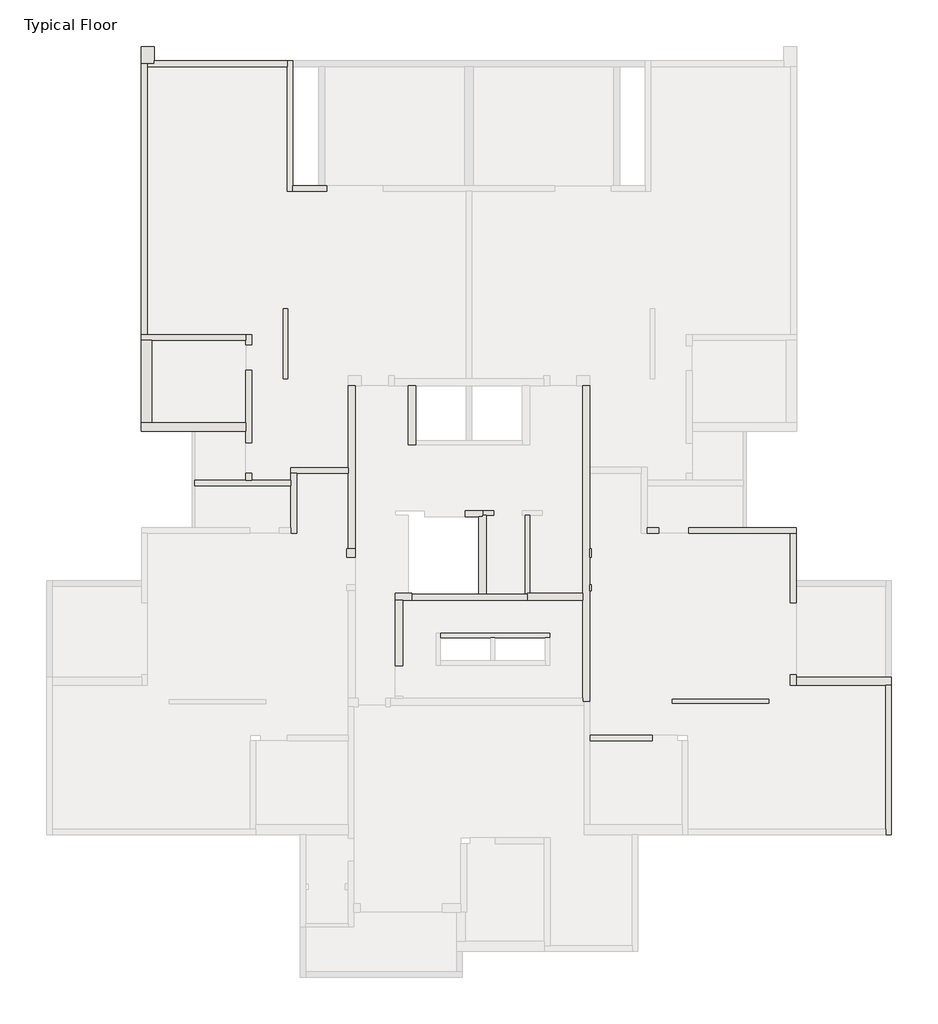
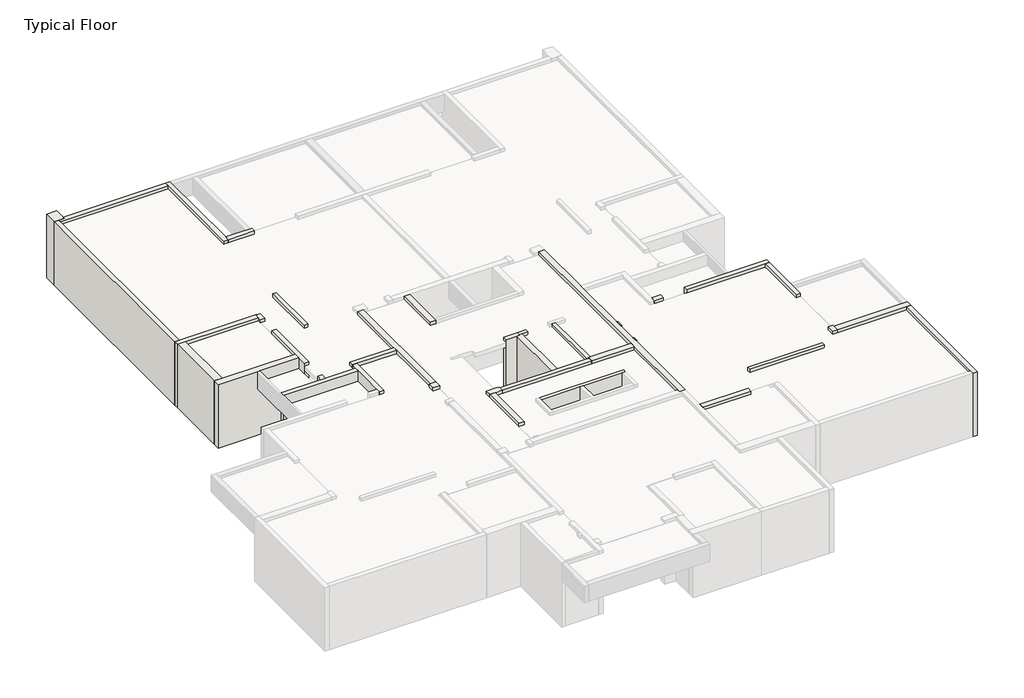
# One storey, part 2 of 4: 38 walls.
"""IFC4 building model written with IfcOpenShell, lengths in millimetres."""

from ifc_helpers import new_model, si_unit, origin, place, context, project, spatial, faceted_brep, element, save

model = new_model("IFC4")

# Units and contexts
model_context = context("Model", 3, world=origin())
ifc_project = project(units=[si_unit("LENGTHUNIT", "METRE", prefix="MILLI")], contexts=[model_context])

# Site, building, storey
site = spatial("IfcSite", under=ifc_project)
building = spatial("IfcBuilding", under=site)
storey = spatial("IfcBuildingStorey", under=building, Name="Typical Floor", Elevation=3160.0)

# Walls
placement = place(None, origin())
element("IfcWall", 1, ObjectType="15", at=placement, inside=storey, context=model_context, shape_type="Brep", body=[
    faceted_brep([(-1883.8880254, 7281.591066, 160.0), (-1883.8880254, 4865.5631538, 160.0), (-1883.8880254, 4865.5631538, 2810.0), (-1883.8880254, 4865.5631538, 3010.0), (-1883.8880254, 4865.5631538, 3160.0), (-1883.8880254, 7281.591066, 3160.0), (-1883.8880254, 7281.591066, 3010.0), (-1883.8880254, 7281.591066, 2810.0), (-1733.8880254, 7281.591066, 160.0), (-1733.8880254, 7281.591066, 2810.0), (-1733.8880254, 7281.591066, 3010.0), (-1733.8880254, 7281.591066, 3160.0), (-1733.8880254, 4865.5631538, 3160.0), (-1733.8880254, 4865.5631538, 3010.0), (-1733.8880254, 4865.5631538, 2810.0), (-1733.8880254, 4865.5631538, 160.0)], [[[0, 1, 2, 3, 4, 5, 6, 7]], [[8, 9, 10, 11, 12, 13, 14, 15]], [[1, 0, 8, 15]], [[4, 3, 2, 1, 15, 14, 13, 12]], [[5, 4, 12, 11]], [[0, 7, 6, 5, 11, 10, 9, 8]]]),
])
element("IfcWall", 2, ObjectType="15", at=placement, inside=storey, context=model_context, shape_type="Brep", body=[
    faceted_brep([(6609.8903055, -2526.1363023, 160.0), (6609.8903055, 156.3601755, 160.0), (6609.8903055, 156.3601755, 2810.0), (6609.8903055, 156.3601755, 3010.0), (6609.8903055, 156.3601755, 3160.0), (6609.8903055, -2526.1363023, 3160.0), (6609.8903055, -2526.1363023, 3010.0), (6609.8903055, -2526.1363023, 2810.0), (6459.8903055, -2576.1363023, 160.0), (6459.8903055, -2576.1363023, 2810.0), (6459.8903055, -2576.1363023, 3010.0), (6459.8903055, -2576.1363023, 3160.0), (6459.8903055, 156.3601755, 3160.0), (6459.8903055, 156.3601755, 3010.0), (6459.8903055, 156.3601755, 2810.0), (6459.8903055, 156.3601755, 160.0), (6534.8903055, -2526.1363023, 160.0), (6534.8903055, -2576.1363023, 160.0), (6534.8903055, -2576.1363023, 3160.0), (6534.8903055, -2526.1363023, 3160.0)], [[[0, 1, 2, 3, 4, 5, 6, 7]], [[8, 9, 10, 11, 12, 13, 14, 15]], [[1, 0, 16, 17, 8, 15]], [[5, 4, 12, 11, 18, 19]], [[0, 7, 6, 5, 19, 16]], [[19, 18, 17, 16]], [[18, 11, 10, 9, 8, 17]], [[4, 3, 2, 1, 15, 14, 13, 12]]]),
])
element("IfcWall", 3, ObjectType="15", at=placement, inside=storey, context=model_context, shape_type="Brep", body=[
    faceted_brep([(11536.8984681, -6331.4817686, 160.0), (14866.281411, -6331.4817686, 160.0), (14866.281411, -6331.4817686, 2810.0), (14866.281411, -6331.4817686, 3010.0), (14866.281411, -6331.4817686, 3160.0), (11536.8984681, -6331.4817686, 3160.0), (11536.8984681, -6331.4817686, 3010.0), (11536.8984681, -6331.4817686, 2810.0), (11536.8984681, -6181.4817686, 160.0), (11536.8984681, -6181.4817686, 2810.0), (11536.8984681, -6181.4817686, 3010.0), (11536.8984681, -6181.4817686, 3160.0), (14866.281411, -6181.4817686, 3160.0), (14866.281411, -6181.4817686, 3010.0), (14866.281411, -6181.4817686, 2810.0), (14866.281411, -6181.4817686, 160.0)], [[[0, 1, 2, 3, 4, 5, 6, 7]], [[8, 9, 10, 11, 12, 13, 14, 15]], [[1, 0, 8, 15]], [[4, 3, 2, 1, 15, 14, 13, 12]], [[5, 4, 12, 11]], [[0, 7, 6, 5, 11, 10, 9, 8]]]),
])
element("IfcWall", 4, ObjectType="15", at=placement, inside=storey, context=model_context, shape_type="Brep", body=[
    faceted_brep([(3535.5549057, -4065.4538564, 160.0), (5268.6420666, -4065.4538564, 160.0), (5418.6420666, -4065.4538564, 160.0), (7154.2538596, -4065.4538564, 160.0), (7304.2538596, -4065.4538564, 160.0), (7304.2538596, -4065.4538564, 3160.0), (7154.2538596, -4065.4538564, 3160.0), (5418.6420666, -4065.4538564, 3160.0), (5268.6420666, -4065.4538564, 3160.0), (3535.5549057, -4065.4538564, 3160.0), (3535.5549057, -3915.4538564, 160.0), (3535.5549057, -3915.4538564, 3160.0), (7304.2538596, -3915.4538564, 3160.0), (7304.2538596, -3915.4538564, 3010.0), (7304.2538596, -3915.4538564, 2810.0), (7304.2538596, -3915.4538564, 160.0)], [[[0, 1, 2, 3, 4, 5, 6, 7, 8, 9]], [[10, 11, 12, 13, 14, 15]], [[4, 3, 2, 1, 0, 10, 15]], [[9, 8, 7, 6, 5, 12, 11]], [[0, 9, 11, 10]], [[5, 4, 15, 14, 13, 12]]]),
])
element("IfcWall", 5, ObjectType="15", at=placement, inside=storey, context=model_context, shape_type="Brep", body=[
    faceted_brep([(4991.7132216, 156.3601755, 160.0), (5116.7132216, 156.3601755, 160.0), (5376.7132216, 156.3601755, 160.0), (5376.7132216, 156.3601755, 2810.0), (5376.7132216, 156.3601755, 3010.0), (5376.7132216, 156.3601755, 3160.0), (5116.7132216, 156.3601755, 3160.0), (4991.7132216, 156.3601755, 3160.0), (4991.7132216, 306.3601755, 160.0), (4991.7132216, 306.3601755, 3160.0), (5376.7132216, 306.3601755, 3160.0), (5376.7132216, 306.3601755, 3010.0), (5376.7132216, 306.3601755, 2810.0), (5376.7132216, 306.3601755, 160.0)], [[[0, 1, 2, 3, 4, 5, 6, 7]], [[8, 9, 10, 11, 12, 13]], [[2, 1, 0, 8, 13]], [[5, 4, 3, 2, 13, 12, 11, 10]], [[7, 6, 5, 10, 9]], [[0, 7, 9, 8]]]),
])
element("IfcWall", 6, ObjectType="20", at=placement, inside=storey, context=model_context, shape_type="Brep", body=[
    faceted_brep([(-6774.1013669, 15724.626844, 160.0), (-6774.1013669, 6387.8215778, 160.0), (-6774.1013669, 6387.8215778, 3160.0), (-6774.1013669, 15724.626844, 3160.0), (-6574.1013669, 15724.626844, 160.0), (-6574.1013669, 15724.626844, 3160.0), (-6574.1013669, 15624.626844, 3160.0), (-6574.1013669, 6387.8215778, 3160.0), (-6574.1013669, 6387.8215778, 3010.0), (-6574.1013669, 6387.8215778, 2810.0), (-6574.1013669, 6387.8215778, 160.0), (-6574.1013669, 15624.626844, 160.0)], [[[0, 1, 2, 3]], [[4, 5, 6, 7, 8, 9, 10, 11]], [[1, 0, 4, 11, 10]], [[3, 2, 7, 6, 5]], [[0, 3, 5, 4]], [[2, 1, 10, 9, 8, 7]]]),
])
element("IfcWall", 7, ObjectType="20", at=placement, inside=storey, context=model_context, shape_type="Brep", body=[
    faceted_brep([(-6774.1013669, 6187.8215778, 160.0), (-6424.1013669, 6187.8215778, 160.0), (-3168.7557226, 6187.8215778, 160.0), (-3168.7557226, 6187.8215778, 2810.0), (-3168.7557226, 6187.8215778, 3010.0), (-3168.7557226, 6187.8215778, 3160.0), (-6424.1013669, 6187.8215778, 3160.0), (-6774.1013669, 6187.8215778, 3160.0), (-6774.1013669, 6387.8215778, 160.0), (-6774.1013669, 6387.8215778, 3160.0), (-6574.1013669, 6387.8215778, 3160.0), (-3168.7557226, 6387.8215778, 3160.0), (-3168.7557226, 6387.8215778, 160.0), (-6574.1013669, 6387.8215778, 160.0)], [[[0, 1, 2, 3, 4, 5, 6, 7]], [[8, 9, 10, 11, 12, 13]], [[2, 1, 0, 8, 13, 12]], [[7, 6, 5, 11, 10, 9]], [[0, 7, 9, 8]], [[5, 4, 3, 2, 12, 11]]]),
])
element("IfcWall", 8, ObjectType="20", at=placement, inside=storey, context=model_context, shape_type="Brep", body=[
    faceted_brep([(-3168.7557226, 1604.6693841, 160.0), (-3168.7557226, 1364.6693841, 160.0), (-3168.7557226, 1364.6693841, 2510.0), (-3168.7557226, 1364.6693841, 2660.0), (-3168.7557226, 1364.6693841, 3160.0), (-3168.7557226, 1604.6693841, 3160.0), (-3168.7557226, 1604.6693841, 3010.0), (-3168.7557226, 1604.6693841, 2810.0), (-2968.7557226, 1604.6693841, 160.0), (-2968.7557226, 1604.6693841, 2810.0), (-2968.7557226, 1604.6693841, 3010.0), (-2968.7557226, 1604.6693841, 3160.0), (-2968.7557226, 1364.6693841, 3160.0), (-2968.7557226, 1364.6693841, 3010.0), (-2968.7557226, 1364.6693841, 2810.0), (-2968.7557226, 1364.6693841, 160.0)], [[[0, 1, 2, 3, 4, 5, 6, 7]], [[8, 9, 10, 11, 12, 13, 14, 15]], [[1, 0, 8, 15]], [[5, 4, 12, 11]], [[0, 7, 6, 5, 11, 10, 9, 8]], [[4, 3, 2, 1, 15, 14, 13, 12]]]),
])
element("IfcWall", 9, ObjectType="20", at=placement, inside=storey, context=model_context, shape_type="Brep", body=[
    faceted_brep([(-1618.0126357, 1364.6693841, 160.0), (-2968.7557226, 1364.6693841, 160.0), (-3168.7557226, 1364.6693841, 160.0), (-4927.8090865, 1364.6693841, 160.0), (-4927.8090865, 1364.6693841, 2510.0), (-4927.8090865, 1364.6693841, 2660.0), (-4927.8090865, 1364.6693841, 3160.0), (-3168.7557226, 1364.6693841, 3160.0), (-2968.7557226, 1364.6693841, 3160.0), (-1618.0126357, 1364.6693841, 3160.0), (-1618.0126357, 1364.6693841, 3010.0), (-1618.0126357, 1364.6693841, 2810.0), (-1618.0126357, 1164.6693841, 160.0), (-1618.0126357, 1164.6693841, 2510.0), (-1618.0126357, 1164.6693841, 2660.0), (-1618.0126357, 1164.6693841, 3160.0), (-4927.8090865, 1164.6693841, 3160.0), (-4927.8090865, 1164.6693841, 2660.0), (-4927.8090865, 1164.6693841, 2510.0), (-4927.8090865, 1164.6693841, 160.0)], [[[0, 1, 2, 3, 4, 5, 6, 7, 8, 9, 10, 11]], [[12, 13, 14, 15, 16, 17, 18, 19]], [[3, 2, 1, 0, 12, 19]], [[6, 5, 4, 3, 19, 18, 17, 16]], [[9, 8, 7, 6, 16, 15]], [[0, 11, 10, 9, 15, 14, 13, 12]]]),
])
element("IfcWall", 10, ObjectType="20", at=placement, inside=storey, context=model_context, shape_type="Brep", body=[
    faceted_brep([(-1750.9499448, 15824.626844, 160.0), (-1750.9499448, 15624.626844, 160.0), (-1750.9499448, 11324.9195447, 160.0), (-1750.9499448, 11324.9195447, 2810.0), (-1750.9499448, 11324.9195447, 3010.0), (-1750.9499448, 11324.9195447, 3160.0), (-1750.9499448, 15624.626844, 3160.0), (-1750.9499448, 15824.626844, 3160.0), (-1550.9499448, 15824.626844, 160.0), (-1550.9499448, 15824.626844, 3160.0), (-1550.9499448, 11524.9195447, 3160.0), (-1550.9499448, 11324.9195447, 3160.0), (-1550.9499448, 11324.9195447, 160.0), (-1550.9499448, 11524.9195447, 160.0)], [[[0, 1, 2, 3, 4, 5, 6, 7]], [[8, 9, 10, 11, 12, 13]], [[2, 1, 0, 8, 13, 12]], [[7, 6, 5, 11, 10, 9]], [[0, 7, 9, 8]], [[5, 4, 3, 2, 12, 11]]]),
])
element("IfcWall", 11, ObjectType="20", at=placement, inside=storey, context=model_context, shape_type="Brep", body=[
    faceted_brep([(-1750.9499448, 15824.626844, 160.0), (-6324.1013669, 15824.626844, 160.0), (-6324.1013669, 15824.626844, 3160.0), (-1750.9499448, 15824.626844, 3160.0), (-1750.9499448, 15624.626844, 160.0), (-1750.9499448, 15624.626844, 2810.0), (-1750.9499448, 15624.626844, 3010.0), (-1750.9499448, 15624.626844, 3160.0), (-6574.1013669, 15624.626844, 3160.0), (-6574.1013669, 15624.626844, 3010.0), (-6574.1013669, 15624.626844, 2810.0), (-6574.1013669, 15624.626844, 160.0), (-6574.1013669, 15724.626844, 160.0), (-6324.1013669, 15724.626844, 160.0), (-6324.1013669, 15724.626844, 3160.0), (-6574.1013669, 15724.626844, 3160.0)], [[[0, 1, 2, 3]], [[4, 5, 6, 7, 8, 9, 10, 11]], [[1, 0, 4, 11, 12, 13]], [[3, 2, 14, 15, 8, 7]], [[0, 3, 7, 6, 5, 4]], [[2, 1, 13, 14]], [[13, 12, 15, 14]], [[12, 11, 10, 9, 8, 15]]]),
])
element("IfcWall", 12, ObjectType="20", at=placement, inside=storey, context=model_context, shape_type="Brep", body=[
    faceted_brep([(15808.1220541, -271.5348131, 160.0), (12108.1220541, -271.5348131, 160.0), (12108.1220541, -271.5348131, 2510.0), (12108.1220541, -271.5348131, 2660.0), (12108.1220541, -271.5348131, 3160.0), (15808.1220541, -271.5348131, 3160.0), (15808.1220541, -471.5348131, 160.0), (15808.1220541, -471.5348131, 3160.0), (15608.1220541, -471.5348131, 3160.0), (12108.1220541, -471.5348131, 3160.0), (12108.1220541, -471.5348131, 2660.0), (12108.1220541, -471.5348131, 2510.0), (12108.1220541, -471.5348131, 160.0), (15608.1220541, -471.5348131, 160.0)], [[[0, 1, 2, 3, 4, 5]], [[6, 7, 8, 9, 10, 11, 12, 13]], [[1, 0, 6, 13, 12]], [[4, 3, 2, 1, 12, 11, 10, 9]], [[5, 4, 9, 8, 7]], [[0, 5, 7, 6]]]),
])
element("IfcWall", 13, ObjectType="20", at=placement, inside=storey, context=model_context, shape_type="Brep", body=[
    faceted_brep([(15608.1220541, -5351.6580536, 160.0), (15608.1220541, -5711.5348131, 160.0), (15608.1220541, -5711.5348131, 2810.0), (15608.1220541, -5711.5348131, 3010.0), (15608.1220541, -5711.5348131, 3160.0), (15608.1220541, -5351.6580536, 3160.0), (15608.1220541, -5351.6580536, 3010.0), (15608.1220541, -5351.6580536, 2810.0), (15808.1220541, -5351.6580536, 160.0), (15808.1220541, -5351.6580536, 2810.0), (15808.1220541, -5351.6580536, 3010.0), (15808.1220541, -5351.6580536, 3160.0), (15808.1220541, -5431.5348131, 3160.0), (15808.1220541, -5711.5348131, 3160.0), (15808.1220541, -5711.5348131, 160.0), (15808.1220541, -5431.5348131, 160.0)], [[[0, 1, 2, 3, 4, 5, 6, 7]], [[8, 9, 10, 11, 12, 13, 14, 15]], [[1, 0, 8, 15, 14]], [[5, 4, 13, 12, 11]], [[0, 7, 6, 5, 11, 10, 9, 8]], [[4, 3, 2, 1, 14, 13]]]),
])
element("IfcWall", 14, ObjectType="20", at=placement, inside=storey, context=model_context, shape_type="Brep", body=[
    faceted_brep([(18889.4302812, -5711.5348131, 160.0), (18889.4302812, -10669.1739201, 160.0), (18889.4302812, -10869.1739201, 160.0), (18889.4302812, -10869.1739201, 3160.0), (18889.4302812, -10669.1739201, 3160.0), (18889.4302812, -5711.5348131, 3160.0), (18889.4302812, -5711.5348131, 3010.0), (18889.4302812, -5711.5348131, 2810.0), (19089.4302812, -5711.5348131, 160.0), (19089.4302812, -5711.5348131, 3160.0), (19089.4302812, -10869.1739201, 3160.0), (19089.4302812, -10869.1739201, 160.0)], [[[0, 1, 2, 3, 4, 5, 6, 7]], [[8, 9, 10, 11]], [[2, 1, 0, 8, 11]], [[5, 4, 3, 10, 9]], [[0, 7, 6, 5, 9, 8]], [[3, 2, 11, 10]]]),
])
element("IfcWall", 15, ObjectType="20", at=placement, inside=storey, context=model_context, shape_type="Brep", body=[
    faceted_brep([(10849.2361919, -7425.251138, 160.0), (8689.2361919, -7425.251138, 160.0), (8689.2361919, -7425.251138, 2810.0), (8689.2361919, -7425.251138, 3010.0), (8689.2361919, -7425.251138, 3160.0), (10849.2361919, -7425.251138, 3160.0), (10849.2361919, -7425.251138, 3010.0), (10849.2361919, -7425.251138, 2810.0), (10849.2361919, -7625.251138, 160.0), (10849.2361919, -7625.251138, 2810.0), (10849.2361919, -7625.251138, 3010.0), (10849.2361919, -7625.251138, 3160.0), (8689.2361919, -7625.251138, 3160.0), (8689.2361919, -7625.251138, 3010.0), (8689.2361919, -7625.251138, 2810.0), (8689.2361919, -7625.251138, 160.0)], [[[0, 1, 2, 3, 4, 5, 6, 7]], [[8, 9, 10, 11, 12, 13, 14, 15]], [[1, 0, 8, 15]], [[5, 4, 12, 11]], [[0, 7, 6, 5, 11, 10, 9, 8]], [[4, 3, 2, 1, 15, 14, 13, 12]]]),
])
element("IfcWall", 16, ObjectType="20", at=placement, inside=storey, context=model_context, shape_type="Brep", body=[
    faceted_brep([(8689.2361919, -2440.6761415, 160.0), (8740.4562765, -2440.6761415, 160.0), (8740.4562765, -2440.6761415, 2810.0), (8740.4562765, -2440.6761415, 3010.0), (8740.4562765, -2440.6761415, 3160.0), (8689.2361919, -2440.6761415, 3160.0), (8689.2361919, -2440.6761415, 3010.0), (8689.2361919, -2440.6761415, 2810.0), (8689.2361919, -2240.6761415, 160.0), (8689.2361919, -2240.6761415, 2810.0), (8689.2361919, -2240.6761415, 3010.0), (8689.2361919, -2240.6761415, 3160.0), (8740.4562765, -2240.6761415, 3160.0), (8740.4562765, -2240.6761415, 3010.0), (8740.4562765, -2240.6761415, 2810.0), (8740.4562765, -2240.6761415, 160.0)], [[[0, 1, 2, 3, 4, 5, 6, 7]], [[8, 9, 10, 11, 12, 13, 14, 15]], [[1, 0, 8, 15]], [[4, 3, 2, 1, 15, 14, 13, 12]], [[5, 4, 12, 11]], [[0, 7, 6, 5, 11, 10, 9, 8]]]),
])
element("IfcWall", 17, ObjectType="20", at=placement, inside=storey, context=model_context, shape_type="Brep", body=[
    faceted_brep([(6534.8903055, -2576.1363023, 160.0), (6459.8903055, -2576.1363023, 160.0), (5116.7132216, -2576.1363023, 160.0), (4866.7132216, -2576.1363023, 160.0), (2556.6955539, -2576.1363023, 160.0), (2556.6955539, -2576.1363023, 3160.0), (2681.6955539, -2576.1363023, 3160.0), (4866.7132216, -2576.1363023, 3160.0), (5116.7132216, -2576.1363023, 3160.0), (6459.8903055, -2576.1363023, 3160.0), (6534.8903055, -2576.1363023, 3160.0), (6534.8903055, -2776.1363023, 160.0), (6534.8903055, -2776.1363023, 3160.0), (2556.6955539, -2776.1363023, 3160.0), (2556.6955539, -2776.1363023, 160.0)], [[[0, 1, 2, 3, 4, 5, 6, 7, 8, 9, 10]], [[11, 12, 13, 14]], [[4, 3, 2, 1, 0, 11, 14]], [[5, 4, 14, 13]], [[10, 9, 8, 7, 6, 5, 13, 12]], [[0, 10, 12, 11]]]),
])
element("IfcWall", 18, ObjectType="20", at=placement, inside=storey, context=model_context, shape_type="Brep", body=[
    faceted_brep([(4391.7132216, 106.3601755, 160.0), (4866.7132216, 106.3601755, 160.0), (4991.7132216, 106.3601755, 160.0), (4991.7132216, 106.3601755, 3160.0), (4866.7132216, 106.3601755, 3160.0), (4391.7132216, 106.3601755, 3160.0), (4391.7132216, 106.3601755, 3010.0), (4391.7132216, 106.3601755, 2810.0), (4391.7132216, 306.3601755, 160.0), (4391.7132216, 306.3601755, 2810.0), (4391.7132216, 306.3601755, 3010.0), (4391.7132216, 306.3601755, 3160.0), (4991.7132216, 306.3601755, 3160.0), (4991.7132216, 306.3601755, 160.0), (4991.7132216, 156.3601755, 160.0), (4991.7132216, 156.3601755, 3160.0)], [[[0, 1, 2, 3, 4, 5, 6, 7]], [[8, 9, 10, 11, 12, 13]], [[2, 1, 0, 8, 13, 14]], [[3, 2, 14, 13, 12, 15]], [[5, 4, 3, 15, 12, 11]], [[0, 7, 6, 5, 11, 10, 9, 8]]]),
])
element("IfcWall", 19, ObjectType="20", at=placement, inside=storey, context=model_context, shape_type="Brep", body=[
    faceted_brep([(-1618.0126357, 1602.0583306, 160.0), (-1418.0126357, 1602.0583306, 160.0), (353.0602083, 1602.0583306, 160.0), (353.0602083, 1602.0583306, 2810.0), (353.0602083, 1602.0583306, 3010.0), (353.0602083, 1602.0583306, 3160.0), (-1418.0126357, 1602.0583306, 3160.0), (-1618.0126357, 1602.0583306, 3160.0), (-1618.0126357, 1802.0583306, 160.0), (-1618.0126357, 1802.0583306, 2810.0), (-1618.0126357, 1802.0583306, 3010.0), (-1618.0126357, 1802.0583306, 3160.0), (353.0602083, 1802.0583306, 3160.0), (353.0602083, 1802.0583306, 3010.0), (353.0602083, 1802.0583306, 2810.0), (353.0602083, 1802.0583306, 160.0)], [[[0, 1, 2, 3, 4, 5, 6, 7]], [[8, 9, 10, 11, 12, 13, 14, 15]], [[2, 1, 0, 8, 15]], [[7, 6, 5, 12, 11]], [[5, 4, 3, 2, 15, 14, 13, 12]], [[0, 7, 11, 10, 9, 8]]]),
])
element("IfcWall", 20, ObjectType="20", at=placement, inside=storey, context=model_context, shape_type="Brep", body=[
    faceted_brep([(-1618.0126357, 1602.0583306, 160.0), (-1618.0126357, 1364.6693841, 160.0), (-1618.0126357, 1164.6693841, 160.0), (-1618.0126357, -271.5347538, 160.0), (-1618.0126357, -471.5347538, 160.0), (-1618.0126357, -471.5347538, 3160.0), (-1618.0126357, -271.5347538, 3160.0), (-1618.0126357, 1164.6693841, 3160.0), (-1618.0126357, 1364.6693841, 3160.0), (-1618.0126357, 1602.0583306, 3160.0), (-1418.0126357, 1602.0583306, 160.0), (-1418.0126357, 1602.0583306, 2810.0), (-1418.0126357, 1602.0583306, 3010.0), (-1418.0126357, 1602.0583306, 3160.0), (-1418.0126357, -471.5347538, 3160.0), (-1418.0126357, -471.5347538, 3010.0), (-1418.0126357, -471.5347538, 2810.0), (-1418.0126357, -471.5347538, 160.0)], [[[0, 1, 2, 3, 4, 5, 6, 7, 8, 9]], [[10, 11, 12, 13, 14, 15, 16, 17]], [[4, 3, 2, 1, 0, 10, 17]], [[9, 8, 7, 6, 5, 14, 13]], [[5, 4, 17, 16, 15, 14]], [[0, 9, 13, 12, 11, 10]]]),
])
element("IfcWall", 21, ObjectType="20", at=placement, inside=storey, context=model_context, shape_type="Brep", body=[
    faceted_brep([(15808.1220541, -2868.5711301, 160.0), (15808.1220541, -471.5348131, 160.0), (15808.1220541, -471.5348131, 3160.0), (15808.1220541, -2868.5711301, 3160.0), (15808.1220541, -2868.5711301, 3010.0), (15808.1220541, -2868.5711301, 2810.0), (15608.1220541, -2868.5711301, 160.0), (15608.1220541, -2868.5711301, 2810.0), (15608.1220541, -2868.5711301, 3010.0), (15608.1220541, -2868.5711301, 3160.0), (15608.1220541, -471.5348131, 3160.0), (15608.1220541, -471.5348131, 3010.0), (15608.1220541, -471.5348131, 2810.0), (15608.1220541, -471.5348131, 160.0)], [[[0, 1, 2, 3, 4, 5]], [[6, 7, 8, 9, 10, 11, 12, 13]], [[1, 0, 6, 13]], [[3, 2, 10, 9]], [[0, 5, 4, 3, 9, 8, 7, 6]], [[2, 1, 13, 12, 11, 10]]]),
])
element("IfcWall", 22, ObjectType="20", at=placement, inside=storey, context=model_context, shape_type="Brep", body=[
    faceted_brep([(-390.7110009, 11524.9195447, 160.0), (-1550.9499448, 11524.9195447, 160.0), (-1550.9499448, 11524.9195447, 3160.0), (-390.7110009, 11524.9195447, 3160.0), (-390.7110009, 11524.9195447, 3010.0), (-390.7110009, 11524.9195447, 2810.0), (-390.7110009, 11324.9195447, 160.0), (-390.7110009, 11324.9195447, 2810.0), (-390.7110009, 11324.9195447, 3010.0), (-390.7110009, 11324.9195447, 3160.0), (-1550.9499448, 11324.9195447, 3160.0), (-1550.9499448, 11324.9195447, 160.0)], [[[0, 1, 2, 3, 4, 5]], [[6, 7, 8, 9, 10, 11]], [[1, 0, 6, 11]], [[3, 2, 10, 9]], [[0, 5, 4, 3, 9, 8, 7, 6]], [[2, 1, 11, 10]]]),
])
element("IfcWall", 23, ObjectType="20", at=placement, inside=storey, context=model_context, shape_type="Brep", body=[
    faceted_brep([(-2968.7557226, 2648.3506111, 160.0), (-2968.7557226, 5158.3506111, 160.0), (-2968.7557226, 5158.3506111, 2810.0), (-2968.7557226, 5158.3506111, 3010.0), (-2968.7557226, 5158.3506111, 3160.0), (-2968.7557226, 2648.3506111, 3160.0), (-2968.7557226, 2648.3506111, 3010.0), (-2968.7557226, 2648.3506111, 2810.0), (-3168.7557226, 2648.3506111, 160.0), (-3168.7557226, 2648.3506111, 2810.0), (-3168.7557226, 2648.3506111, 3010.0), (-3168.7557226, 2648.3506111, 3160.0), (-3168.7557226, 3048.3506111, 3160.0), (-3168.7557226, 3348.3506111, 3160.0), (-3168.7557226, 5158.3506111, 3160.0), (-3168.7557226, 5158.3506111, 3010.0), (-3168.7557226, 5158.3506111, 2810.0), (-3168.7557226, 5158.3506111, 160.0), (-3168.7557226, 3348.3506111, 160.0), (-3168.7557226, 3048.3506111, 160.0)], [[[0, 1, 2, 3, 4, 5, 6, 7]], [[8, 9, 10, 11, 12, 13, 14, 15, 16, 17, 18, 19]], [[1, 0, 8, 19, 18, 17]], [[4, 3, 2, 1, 17, 16, 15, 14]], [[5, 4, 14, 13, 12, 11]], [[0, 7, 6, 5, 11, 10, 9, 8]]]),
])
element("IfcWall", 24, ObjectType="20", at=placement, inside=storey, context=model_context, shape_type="Brep", body=[
    faceted_brep([(-3168.7557226, 6387.8215778, 160.0), (-3168.7557226, 6187.8215778, 160.0), (-3168.7557226, 6027.8215778, 160.0), (-3168.7557226, 6027.8215778, 2810.0), (-3168.7557226, 6027.8215778, 3010.0), (-3168.7557226, 6027.8215778, 3160.0), (-3168.7557226, 6187.8215778, 3160.0), (-3168.7557226, 6387.8215778, 3160.0), (-2968.7557226, 6387.8215778, 160.0), (-2968.7557226, 6387.8215778, 2810.0), (-2968.7557226, 6387.8215778, 3010.0), (-2968.7557226, 6387.8215778, 3160.0), (-2968.7557226, 6027.8215778, 3160.0), (-2968.7557226, 6027.8215778, 3010.0), (-2968.7557226, 6027.8215778, 2810.0), (-2968.7557226, 6027.8215778, 160.0)], [[[0, 1, 2, 3, 4, 5, 6, 7]], [[8, 9, 10, 11, 12, 13, 14, 15]], [[2, 1, 0, 8, 15]], [[5, 4, 3, 2, 15, 14, 13, 12]], [[7, 6, 5, 12, 11]], [[0, 7, 11, 10, 9, 8]]]),
])
element("IfcWall", 25, ObjectType="20", at=placement, inside=storey, context=model_context, shape_type="Brep", body=[
    faceted_brep([(11062.1205752, -271.5348131, 160.0), (10662.1205752, -271.5348131, 160.0), (10662.1205752, -271.5348131, 2510.0), (10662.1205752, -271.5348131, 2660.0), (10662.1205752, -271.5348131, 3160.0), (11062.1205752, -271.5348131, 3160.0), (11062.1205752, -271.5348131, 2660.0), (11062.1205752, -271.5348131, 2510.0), (11062.1205752, -471.5348131, 160.0), (11062.1205752, -471.5348131, 2510.0), (11062.1205752, -471.5348131, 2660.0), (11062.1205752, -471.5348131, 3160.0), (10662.1205752, -471.5348131, 3160.0), (10662.1205752, -471.5348131, 160.0)], [[[0, 1, 2, 3, 4, 5, 6, 7]], [[8, 9, 10, 11, 12, 13]], [[1, 0, 8, 13]], [[5, 4, 12, 11]], [[0, 7, 6, 5, 11, 10, 9, 8]], [[4, 3, 2, 1, 13, 12]]]),
])
element("IfcWall", 26, ObjectType="25", at=placement, inside=storey, context=model_context, shape_type="Brep", body=[
    faceted_brep([(2434.2185243, 4615.5631538, 160.0), (2434.2185243, 2582.4743311, 160.0), (2434.2185243, 2582.4743311, 2810.0), (2434.2185243, 2582.4743311, 3010.0), (2434.2185243, 2582.4743311, 3160.0), (2434.2185243, 4615.5631538, 3160.0), (2434.2185243, 4615.5631538, 3010.0), (2434.2185243, 4615.5631538, 2810.0), (2684.2185243, 4615.5631538, 160.0), (2684.2185243, 4615.5631538, 3160.0), (2684.2185243, 2732.4743311, 3160.0), (2684.2185243, 2582.4743311, 3160.0), (2684.2185243, 2582.4743311, 160.0), (2684.2185243, 2732.4743311, 160.0)], [[[0, 1, 2, 3, 4, 5, 6, 7]], [[8, 9, 10, 11, 12, 13]], [[1, 0, 8, 13, 12]], [[5, 4, 11, 10, 9]], [[0, 7, 6, 5, 9, 8]], [[4, 3, 2, 1, 12, 11]]]),
])
element("IfcWall", 27, ObjectType="25", at=placement, inside=storey, context=model_context, shape_type="Brep", body=[
    faceted_brep([(8689.2361919, -6275.4733638, 160.0), (8689.2361919, -2440.6761415, 160.0), (8689.2361919, -2240.6761415, 160.0), (8689.2361919, -1298.8355577, 160.0), (8689.2361919, -998.8355577, 160.0), (8689.2361919, 1602.6523966, 160.0), (8689.2361919, 1802.6523966, 160.0), (8689.2361919, 4613.0861241, 160.0), (8689.2361919, 4613.0861241, 3160.0), (8689.2361919, 1802.6523966, 3160.0), (8689.2361919, 1602.6523966, 3160.0), (8689.2361919, -998.8355577, 3160.0), (8689.2361919, -1298.8355577, 3160.0), (8689.2361919, -2240.6761415, 3160.0), (8689.2361919, -2440.6761415, 3160.0), (8689.2361919, -6275.4733638, 3160.0), (8439.2361919, -6275.4733638, 160.0), (8439.2361919, -6275.4733638, 3160.0), (8439.2361919, -6150.4733638, 3160.0), (8439.2361919, -2776.1363023, 3160.0), (8439.2361919, -2526.1363023, 3160.0), (8439.2361919, 4613.0861241, 3160.0), (8439.2361919, 4613.0861241, 3010.0), (8439.2361919, 4613.0861241, 2810.0), (8439.2361919, 4613.0861241, 160.0), (8439.2361919, -2526.1363023, 160.0), (8439.2361919, -2776.1363023, 160.0), (8439.2361919, -6150.4733638, 160.0), (8489.2361919, -6275.4733638, 160.0), (8489.2361919, -6275.4733638, 3160.0)], [[[0, 1, 2, 3, 4, 5, 6, 7, 8, 9, 10, 11, 12, 13, 14, 15]], [[16, 17, 18, 19, 20, 21, 22, 23, 24, 25, 26, 27]], [[7, 6, 5, 4, 3, 2, 1, 0, 28, 16, 27, 26, 25, 24]], [[8, 7, 24, 23, 22, 21]], [[15, 14, 13, 12, 11, 10, 9, 8, 21, 20, 19, 18, 17, 29]], [[0, 15, 29, 17, 16, 28]]]),
])
element("IfcWall", 28, ObjectType="25", at=placement, inside=storey, context=model_context, shape_type="Brep", body=[
    faceted_brep([(8439.2361919, -2526.1363023, 160.0), (6609.8903055, -2526.1363023, 160.0), (6534.8903055, -2526.1363023, 160.0), (6534.8903055, -2526.1363023, 3160.0), (6609.8903055, -2526.1363023, 3160.0), (8439.2361919, -2526.1363023, 3160.0), (8439.2361919, -2526.1363023, 3010.0), (8439.2361919, -2526.1363023, 2810.0), (8439.2361919, -2776.1363023, 160.0), (8439.2361919, -2776.1363023, 3160.0), (6534.8903055, -2776.1363023, 3160.0), (6534.8903055, -2776.1363023, 160.0), (6534.8903055, -2576.1363023, 160.0), (6534.8903055, -2576.1363023, 3160.0)], [[[0, 1, 2, 3, 4, 5, 6, 7]], [[8, 9, 10, 11]], [[2, 1, 0, 8, 11, 12]], [[3, 2, 12, 11, 10, 13]], [[5, 4, 3, 13, 10, 9]], [[0, 7, 6, 5, 9, 8]]]),
])
element("IfcWall", 29, ObjectType="25", at=placement, inside=storey, context=model_context, shape_type="Brep", body=[
    faceted_brep([(4866.7132216, 106.3601755, 160.0), (4866.7132216, -2576.1363023, 160.0), (4866.7132216, -2576.1363023, 3160.0), (4866.7132216, 106.3601755, 3160.0), (5116.7132216, 156.3601755, 160.0), (5116.7132216, 156.3601755, 2810.0), (5116.7132216, 156.3601755, 3010.0), (5116.7132216, 156.3601755, 3160.0), (5116.7132216, -2576.1363023, 3160.0), (5116.7132216, -2576.1363023, 3010.0), (5116.7132216, -2576.1363023, 2810.0), (5116.7132216, -2576.1363023, 160.0), (4991.7132216, 106.3601755, 160.0), (4991.7132216, 156.3601755, 160.0), (4991.7132216, 156.3601755, 3160.0), (4991.7132216, 106.3601755, 3160.0)], [[[0, 1, 2, 3]], [[4, 5, 6, 7, 8, 9, 10, 11]], [[1, 0, 12, 13, 4, 11]], [[3, 2, 8, 7, 14, 15]], [[2, 1, 11, 10, 9, 8]], [[0, 3, 15, 12]], [[15, 14, 13, 12]], [[14, 7, 6, 5, 4, 13]]]),
])
element("IfcWall", 30, ObjectType="25", at=placement, inside=storey, context=model_context, shape_type="Brep", body=[
    faceted_brep([(353.0602083, 4618.0861241, 160.0), (353.0602083, 1802.0583306, 160.0), (353.0602083, 1602.0583306, 160.0), (353.0602083, -998.8355577, 160.0), (353.0602083, -998.8355577, 2810.0), (353.0602083, -998.8355577, 3010.0), (353.0602083, -998.8355577, 3160.0), (353.0602083, 1602.0583306, 3160.0), (353.0602083, 1802.0583306, 3160.0), (353.0602083, 4618.0861241, 3160.0), (603.0602083, 4618.0861241, 160.0), (603.0602083, 4618.0861241, 2810.0), (603.0602083, 4618.0861241, 3010.0), (603.0602083, 4618.0861241, 3160.0), (603.0602083, -998.8355577, 3160.0), (603.0602083, -998.8355577, 160.0)], [[[0, 1, 2, 3, 4, 5, 6, 7, 8, 9]], [[10, 11, 12, 13, 14, 15]], [[3, 2, 1, 0, 10, 15]], [[9, 8, 7, 6, 14, 13]], [[0, 9, 13, 12, 11, 10]], [[6, 5, 4, 3, 15, 14]]]),
])
element("IfcWall", 31, ObjectType="25", at=placement, inside=storey, context=model_context, shape_type="Brep", body=[
    faceted_brep([(2237.3338395, -5031.1363023, 160.0), (2237.3338395, -2776.1363023, 160.0), (2237.3338395, -2776.1363023, 2810.0), (2237.3338395, -2776.1363023, 3010.0), (2237.3338395, -2776.1363023, 3160.0), (2237.3338395, -5031.1363023, 3160.0), (2237.3338395, -5031.1363023, 3010.0), (2237.3338395, -5031.1363023, 2810.0), (1987.3338395, -5031.1363023, 160.0), (1987.3338395, -5031.1363023, 2810.0), (1987.3338395, -5031.1363023, 3010.0), (1987.3338395, -5031.1363023, 3160.0), (1987.3338395, -2776.1363023, 3160.0), (1987.3338395, -2776.1363023, 160.0)], [[[0, 1, 2, 3, 4, 5, 6, 7]], [[8, 9, 10, 11, 12, 13]], [[1, 0, 8, 13]], [[5, 4, 12, 11]], [[0, 7, 6, 5, 11, 10, 9, 8]], [[4, 3, 2, 1, 13, 12]]]),
])
element("IfcWall", 32, ObjectType="25", at=placement, inside=storey, context=model_context, shape_type="Brep", body=[
    faceted_brep([(1987.3338395, -2776.1363023, 160.0), (2237.3338395, -2776.1363023, 160.0), (2556.6955539, -2776.1363023, 160.0), (2556.6955539, -2776.1363023, 3160.0), (2237.3338395, -2776.1363023, 3160.0), (1987.3338395, -2776.1363023, 3160.0), (1987.3338395, -2526.1363023, 160.0), (1987.3338395, -2526.1363023, 2810.0), (1987.3338395, -2526.1363023, 3010.0), (1987.3338395, -2526.1363023, 3160.0), (2431.6955539, -2526.1363023, 3160.0), (2556.6955539, -2526.1363023, 3160.0), (2556.6955539, -2526.1363023, 160.0), (2556.6955539, -2576.1363023, 160.0), (2556.6955539, -2576.1363023, 3160.0)], [[[0, 1, 2, 3, 4, 5]], [[6, 7, 8, 9, 10, 11, 12]], [[2, 1, 0, 6, 12, 13]], [[3, 2, 13, 12, 11, 14]], [[5, 4, 3, 14, 11, 10, 9]], [[0, 5, 9, 8, 7, 6]]]),
])
element("IfcWall", 33, ObjectType="28", at=placement, inside=storey, context=model_context, shape_type="Brep", body=[
    faceted_brep([(15808.1220541, -5711.5348131, 160.0), (18889.4302812, -5711.5348131, 160.0), (19089.4302812, -5711.5348131, 160.0), (19089.4302812, -5711.5348131, 3160.0), (18889.4302812, -5711.5348131, 3160.0), (15808.1220541, -5711.5348131, 3160.0), (15808.1220541, -5431.5348131, 160.0), (15808.1220541, -5431.5348131, 2810.0), (15808.1220541, -5431.5348131, 3010.0), (15808.1220541, -5431.5348131, 3160.0), (19089.4302812, -5431.5348131, 3160.0), (19089.4302812, -5431.5348131, 160.0)], [[[0, 1, 2, 3, 4, 5]], [[6, 7, 8, 9, 10, 11]], [[2, 1, 0, 6, 11]], [[5, 4, 3, 10, 9]], [[0, 5, 9, 8, 7, 6]], [[3, 2, 11, 10]]]),
])
element("IfcWall", 34, ObjectType="30", at=placement, inside=storey, context=model_context, shape_type="Brep", body=[
    faceted_brep([(-3168.7557226, 3348.3506111, 160.0), (-6424.1013669, 3348.3506111, 160.0), (-6774.1013669, 3348.3506111, 160.0), (-6774.1013669, 3348.3506111, 3160.0), (-6424.1013669, 3348.3506111, 3160.0), (-3168.7557226, 3348.3506111, 3160.0), (-3168.7557226, 3348.3506111, 3010.0), (-3168.7557226, 3348.3506111, 2810.0), (-3168.7557226, 3048.3506111, 160.0), (-3168.7557226, 3048.3506111, 2510.0), (-3168.7557226, 3048.3506111, 2660.0), (-3168.7557226, 3048.3506111, 3160.0), (-6774.1013669, 3048.3506111, 3160.0), (-6774.1013669, 3048.3506111, 160.0)], [[[0, 1, 2, 3, 4, 5, 6, 7]], [[8, 9, 10, 11, 12, 13]], [[2, 1, 0, 8, 13]], [[5, 4, 3, 12, 11]], [[3, 2, 13, 12]], [[0, 7, 6, 5, 11, 10, 9, 8]]]),
])
element("IfcWall", 35, ObjectType="30", at=placement, inside=storey, context=model_context, shape_type="Brep", body=[
    faceted_brep([(303.6507728, -1298.8355577, 160.0), (603.0602083, -1298.8355577, 160.0), (603.0602083, -1298.8355577, 2810.0), (603.0602083, -1298.8355577, 3010.0), (603.0602083, -1298.8355577, 3160.0), (303.6507728, -1298.8355577, 3160.0), (303.6507728, -1298.8355577, 3010.0), (303.6507728, -1298.8355577, 2810.0), (303.6507728, -998.8355577, 160.0), (303.6507728, -998.8355577, 2810.0), (303.6507728, -998.8355577, 3010.0), (303.6507728, -998.8355577, 3160.0), (353.0602083, -998.8355577, 3160.0), (603.0602083, -998.8355577, 3160.0), (603.0602083, -998.8355577, 160.0), (353.0602083, -998.8355577, 160.0)], [[[0, 1, 2, 3, 4, 5, 6, 7]], [[8, 9, 10, 11, 12, 13, 14, 15]], [[1, 0, 8, 15, 14]], [[5, 4, 13, 12, 11]], [[0, 7, 6, 5, 11, 10, 9, 8]], [[4, 3, 2, 1, 14, 13]]]),
])
element("IfcWall", 36, ObjectType="30", at=placement, inside=storey, context=model_context, shape_type="Brep", body=[
    faceted_brep([(8689.2361919, -1298.8355577, 160.0), (8740.4562765, -1298.8355577, 160.0), (8740.4562765, -1298.8355577, 2810.0), (8740.4562765, -1298.8355577, 3010.0), (8740.4562765, -1298.8355577, 3160.0), (8689.2361919, -1298.8355577, 3160.0), (8689.2361919, -1298.8355577, 3010.0), (8689.2361919, -1298.8355577, 2810.0), (8689.2361919, -998.8355577, 160.0), (8689.2361919, -998.8355577, 2810.0), (8689.2361919, -998.8355577, 3010.0), (8689.2361919, -998.8355577, 3160.0), (8740.4562765, -998.8355577, 3160.0), (8740.4562765, -998.8355577, 3010.0), (8740.4562765, -998.8355577, 2810.0), (8740.4562765, -998.8355577, 160.0)], [[[0, 1, 2, 3, 4, 5, 6, 7]], [[8, 9, 10, 11, 12, 13, 14, 15]], [[1, 0, 8, 15]], [[4, 3, 2, 1, 15, 14, 13, 12]], [[5, 4, 12, 11]], [[0, 7, 6, 5, 11, 10, 9, 8]]]),
])
element("IfcWall", 37, ObjectType="35", at=placement, inside=storey, context=model_context, shape_type="Brep", body=[
    faceted_brep([(-6424.1013669, 3348.3506111, 160.0), (-6424.1013669, 6187.8215778, 160.0), (-6424.1013669, 6187.8215778, 2810.0), (-6424.1013669, 6187.8215778, 3010.0), (-6424.1013669, 6187.8215778, 3160.0), (-6424.1013669, 3348.3506111, 3160.0), (-6424.1013669, 3348.3506111, 3010.0), (-6424.1013669, 3348.3506111, 2810.0), (-6774.1013669, 3348.3506111, 160.0), (-6774.1013669, 3348.3506111, 3160.0), (-6774.1013669, 6187.8215778, 3160.0), (-6774.1013669, 6187.8215778, 160.0)], [[[0, 1, 2, 3, 4, 5, 6, 7]], [[8, 9, 10, 11]], [[1, 0, 8, 11]], [[5, 4, 10, 9]], [[4, 3, 2, 1, 11, 10]], [[0, 7, 6, 5, 9, 8]]]),
])
element("IfcWall", 38, ObjectType="45", at=placement, inside=storey, context=model_context, shape_type="Brep", body=[
    faceted_brep([(-6774.1013669, 16318.9904575, 160.0), (-6774.1013669, 15724.626844, 160.0), (-6774.1013669, 15724.626844, 3160.0), (-6774.1013669, 16318.9904575, 3160.0), (-6324.1013669, 16318.9904575, 160.0), (-6324.1013669, 16318.9904575, 3160.0), (-6324.1013669, 15824.626844, 3160.0), (-6324.1013669, 15724.626844, 3160.0), (-6324.1013669, 15724.626844, 160.0), (-6324.1013669, 15824.626844, 160.0), (-6574.1013669, 15724.626844, 160.0), (-6574.1013669, 15724.626844, 3160.0)], [[[0, 1, 2, 3]], [[4, 5, 6, 7, 8, 9]], [[1, 0, 4, 9, 8, 10]], [[2, 1, 10, 8, 7, 11]], [[3, 2, 11, 7, 6, 5]], [[0, 3, 5, 4]]]),
])

save(model, "model.ifc")

# Revit data of these elements
# Type "15"
#   Layers, outside or top first: 15 cm "Concrete, Cast-in-Place - B30" (function 1)
# Type "20"
#   Layers, outside or top first: 20 cm "Concrete, Cast-in-Place - B30" (function 1)
# Type "25"
#   Layers, outside or top first: 25 cm "Concrete, Cast-in-Place - B30" (function 1)
# Type "28"
#   Layers, outside or top first: 28 cm "Concrete, Cast-in-Place - B30" (function 1)
# Type "30"
#   Layers, outside or top first: 30 cm "Concrete, Cast-in-Place - B30" (function 1)
# Type "35"
#   Layers, outside or top first: 35 cm "Concrete, Cast-in-Place - B30" (function 1)
# Type "45"
#   Layers, outside or top first: 45 cm "Concrete, Cast-in-Place - B30" (function 1)
# Element 1 (IfcWall, "15")
#   Comments = ""
#   Mark = "W92"
#   SOFiSTiK_AMG_Comments = ""
#   built-in parameter 1001111 = -300 cm
#   Top Offset = 0 cm
#   Base Offset = -300 cm
#   wall height = 300 cm
#   SOFiSTiK_AMG_Scheduled = yes
#   SOFiSTiK_AMG_Adjusted = yes
#   Phase Created = New Construction
#   Base Constraint = Typical Floor
#   Top Constraint = Typical Floor
#   Materials on its faces: "Concrete, Cast-in-Place - B30"
# Element 2 (IfcWall, "15")
#   Comments = ""
#   Mark = "W93"
#   SOFiSTiK_AMG_Comments = ""
#   built-in parameter 1001111 = -300 cm
#   Top Offset = 0 cm
#   Base Offset = -300 cm
#   wall height = 300 cm
#   SOFiSTiK_AMG_Scheduled = yes
#   SOFiSTiK_AMG_Adjusted = yes
#   Phase Created = New Construction
#   Base Constraint = Typical Floor
#   Top Constraint = Typical Floor
#   Materials on its faces: "Concrete, Cast-in-Place - B30"
# Element 3 (IfcWall, "15")
#   Comments = ""
#   Mark = "W97"
#   SOFiSTiK_AMG_Comments = ""
#   built-in parameter 1001111 = -300 cm
#   Top Offset = 0 cm
#   Base Offset = -300 cm
#   wall height = 300 cm
#   SOFiSTiK_AMG_Scheduled = yes
#   SOFiSTiK_AMG_Adjusted = yes
#   Phase Created = New Construction
#   Base Constraint = Typical Floor
#   Top Constraint = Typical Floor
#   Materials on its faces: "Concrete, Cast-in-Place - B30"
# Element 4 (IfcWall, "15")
#   Comments = ""
#   Mark = "W99"
#   SOFiSTiK_AMG_Comments = ""
#   built-in parameter 1001111 = -300 cm
#   Top Offset = 0 cm
#   Base Offset = -300 cm
#   wall height = 300 cm
#   SOFiSTiK_AMG_Scheduled = yes
#   SOFiSTiK_AMG_Adjusted = yes
#   Phase Created = New Construction
#   Base Constraint = Typical Floor
#   Top Constraint = Typical Floor
#   Materials on its faces: "Concrete, Cast-in-Place - B30"
# Element 5 (IfcWall, "15")
#   Comments = ""
#   Mark = "W103"
#   SOFiSTiK_AMG_Comments = ""
#   built-in parameter 1001111 = -300 cm
#   Top Offset = 0 cm
#   Base Offset = -300 cm
#   wall height = 300 cm
#   SOFiSTiK_AMG_Scheduled = yes
#   SOFiSTiK_AMG_Adjusted = yes
#   Phase Created = New Construction
#   Base Constraint = Typical Floor
#   Top Constraint = Typical Floor
#   Materials on its faces: "Concrete, Cast-in-Place - B30"
# Element 6 (IfcWall, "20")
#   Comments = ""
#   Mark = "W1"
#   SOFiSTiK_AMG_Comments = ""
#   built-in parameter 1001111 = -300 cm
#   Top Offset = 0 cm
#   Base Offset = -300 cm
#   wall height = 300 cm
#   SOFiSTiK_AMG_Scheduled = yes
#   SOFiSTiK_AMG_Adjusted = yes
#   Phase Created = New Construction
#   Base Constraint = Typical Floor
#   Top Constraint = Typical Floor
#   Materials on its faces: "Concrete, Cast-in-Place - B30"
# Element 7 (IfcWall, "20")
#   Comments = ""
#   Mark = "W2"
#   SOFiSTiK_AMG_Comments = ""
#   built-in parameter 1001111 = -300 cm
#   Top Offset = 0 cm
#   Base Offset = -300 cm
#   wall height = 300 cm
#   SOFiSTiK_AMG_Scheduled = yes
#   SOFiSTiK_AMG_Adjusted = yes
#   Phase Created = New Construction
#   Base Constraint = Typical Floor
#   Top Constraint = Typical Floor
#   Materials on its faces: "Concrete, Cast-in-Place - B30"
# Element 8 (IfcWall, "20")
#   Comments = ""
#   Mark = "W3"
#   SOFiSTiK_AMG_Comments = ""
#   built-in parameter 1001111 = -300 cm
#   Top Offset = 0 cm
#   Base Offset = -300 cm
#   wall height = 300 cm
#   SOFiSTiK_AMG_Scheduled = yes
#   SOFiSTiK_AMG_Adjusted = yes
#   Phase Created = New Construction
#   Base Constraint = Typical Floor
#   Top Constraint = Typical Floor
#   Materials on its faces: "Concrete, Cast-in-Place - B30"
# Element 9 (IfcWall, "20")
#   Comments = ""
#   Mark = "W4"
#   SOFiSTiK_AMG_Comments = ""
#   built-in parameter 1001111 = -300 cm
#   Top Offset = 0 cm
#   Base Offset = -300 cm
#   wall height = 300 cm
#   SOFiSTiK_AMG_Scheduled = yes
#   SOFiSTiK_AMG_Adjusted = yes
#   Phase Created = New Construction
#   Base Constraint = Typical Floor
#   Top Constraint = Typical Floor
#   Materials on its faces: "Concrete, Cast-in-Place - B30"
# Element 10 (IfcWall, "20")
#   Comments = ""
#   Mark = "W5"
#   SOFiSTiK_AMG_Comments = ""
#   built-in parameter 1001111 = -300 cm
#   Top Offset = 0 cm
#   Base Offset = -300 cm
#   wall height = 300 cm
#   SOFiSTiK_AMG_Scheduled = yes
#   SOFiSTiK_AMG_Adjusted = yes
#   Phase Created = New Construction
#   Base Constraint = Typical Floor
#   Top Constraint = Typical Floor
#   Materials on its faces: "Concrete, Cast-in-Place - B30"
# Element 11 (IfcWall, "20")
#   Comments = ""
#   Mark = "W11"
#   SOFiSTiK_AMG_Comments = ""
#   built-in parameter 1001111 = -300 cm
#   Top Offset = 0 cm
#   Base Offset = -300 cm
#   wall height = 300 cm
#   SOFiSTiK_AMG_Scheduled = yes
#   SOFiSTiK_AMG_Adjusted = yes
#   Phase Created = New Construction
#   Base Constraint = Typical Floor
#   Top Constraint = Typical Floor
#   Materials on its faces: "Concrete, Cast-in-Place - B30"
# Element 12 (IfcWall, "20")
#   Comments = ""
#   Mark = "W22"
#   SOFiSTiK_AMG_Comments = ""
#   built-in parameter 1001111 = -300 cm
#   Top Offset = 0 cm
#   Base Offset = -300 cm
#   wall height = 300 cm
#   SOFiSTiK_AMG_Scheduled = yes
#   SOFiSTiK_AMG_Adjusted = yes
#   Phase Created = New Construction
#   Base Constraint = Typical Floor
#   Top Constraint = Typical Floor
#   Materials on its faces: "Concrete, Cast-in-Place - B30"
# Element 13 (IfcWall, "20")
#   Comments = ""
#   Mark = "W23"
#   SOFiSTiK_AMG_Comments = ""
#   built-in parameter 1001111 = -300 cm
#   Top Offset = 0 cm
#   Base Offset = -300 cm
#   wall height = 300 cm
#   SOFiSTiK_AMG_Scheduled = yes
#   SOFiSTiK_AMG_Adjusted = yes
#   Phase Created = New Construction
#   Base Constraint = Typical Floor
#   Top Constraint = Typical Floor
#   Materials on its faces: "Concrete, Cast-in-Place - B30"
# Element 14 (IfcWall, "20")
#   Comments = ""
#   Mark = "W24"
#   SOFiSTiK_AMG_Comments = ""
#   built-in parameter 1001111 = -300 cm
#   Top Offset = 0 cm
#   Base Offset = -300 cm
#   wall height = 300 cm
#   SOFiSTiK_AMG_Scheduled = yes
#   SOFiSTiK_AMG_Adjusted = yes
#   Phase Created = New Construction
#   Base Constraint = Typical Floor
#   Top Constraint = Typical Floor
#   Materials on its faces: "Concrete, Cast-in-Place - B30"
# Element 15 (IfcWall, "20")
#   Comments = ""
#   Mark = "W27"
#   SOFiSTiK_AMG_Comments = ""
#   built-in parameter 1001111 = -300 cm
#   Top Offset = 0 cm
#   Base Offset = -300 cm
#   wall height = 300 cm
#   SOFiSTiK_AMG_Scheduled = yes
#   SOFiSTiK_AMG_Adjusted = yes
#   Phase Created = New Construction
#   Base Constraint = Typical Floor
#   Top Constraint = Typical Floor
#   Materials on its faces: "Concrete, Cast-in-Place - B30"
# Element 16 (IfcWall, "20")
#   Comments = ""
#   Mark = "W29"
#   SOFiSTiK_AMG_Comments = "Too Short /"
#   built-in parameter 1001111 = -300 cm
#   Top Offset = 0 cm
#   Base Offset = -300 cm
#   wall height = 300 cm
#   SOFiSTiK_AMG_Scheduled = yes
#   SOFiSTiK_AMG_Adjusted = yes
#   Phase Created = New Construction
#   Base Constraint = Typical Floor
#   Top Constraint = Typical Floor
#   Materials on its faces: "Concrete, Cast-in-Place - B30"
# Element 17 (IfcWall, "20")
#   Comments = ""
#   Mark = "W30"
#   SOFiSTiK_AMG_Comments = ""
#   built-in parameter 1001111 = -300 cm
#   Top Offset = 0 cm
#   Base Offset = -300 cm
#   wall height = 300 cm
#   SOFiSTiK_AMG_Scheduled = yes
#   SOFiSTiK_AMG_Adjusted = yes
#   Phase Created = New Construction
#   Base Constraint = Typical Floor
#   Top Constraint = Typical Floor
#   Materials on its faces: "Concrete, Cast-in-Place - B30"
# Element 18 (IfcWall, "20")
#   Comments = ""
#   Mark = "W31"
#   SOFiSTiK_AMG_Comments = ""
#   built-in parameter 1001111 = -300 cm
#   Top Offset = 0 cm
#   Base Offset = -300 cm
#   wall height = 300 cm
#   SOFiSTiK_AMG_Scheduled = yes
#   SOFiSTiK_AMG_Adjusted = yes
#   Phase Created = New Construction
#   Base Constraint = Typical Floor
#   Top Constraint = Typical Floor
#   Materials on its faces: "Concrete, Cast-in-Place - B30"
# Element 19 (IfcWall, "20")
#   Comments = ""
#   Mark = "W32"
#   SOFiSTiK_AMG_Comments = ""
#   built-in parameter 1001111 = -300 cm
#   Top Offset = 0 cm
#   Base Offset = -300 cm
#   wall height = 300 cm
#   SOFiSTiK_AMG_Scheduled = yes
#   SOFiSTiK_AMG_Adjusted = yes
#   Phase Created = New Construction
#   Base Constraint = Typical Floor
#   Top Constraint = Typical Floor
#   Materials on its faces: "Concrete, Cast-in-Place - B30"
# Element 20 (IfcWall, "20")
#   Comments = ""
#   Mark = "W33"
#   SOFiSTiK_AMG_Comments = ""
#   built-in parameter 1001111 = -300 cm
#   Top Offset = 0 cm
#   Base Offset = -300 cm
#   wall height = 300 cm
#   SOFiSTiK_AMG_Scheduled = yes
#   SOFiSTiK_AMG_Adjusted = yes
#   Phase Created = New Construction
#   Base Constraint = Typical Floor
#   Top Constraint = Typical Floor
#   Materials on its faces: "Concrete, Cast-in-Place - B30"
# Element 21 (IfcWall, "20")
#   Comments = ""
#   Mark = "W46"
#   SOFiSTiK_AMG_Comments = ""
#   built-in parameter 1001111 = -300 cm
#   Top Offset = 0 cm
#   Base Offset = -300 cm
#   wall height = 300 cm
#   SOFiSTiK_AMG_Scheduled = yes
#   SOFiSTiK_AMG_Adjusted = yes
#   Phase Created = New Construction
#   Base Constraint = Typical Floor
#   Top Constraint = Typical Floor
#   Materials on its faces: "Concrete, Cast-in-Place - B30"
# Element 22 (IfcWall, "20")
#   Comments = ""
#   Mark = "W50"
#   SOFiSTiK_AMG_Comments = ""
#   built-in parameter 1001111 = -300 cm
#   Top Offset = 0 cm
#   Base Offset = -300 cm
#   wall height = 300 cm
#   SOFiSTiK_AMG_Scheduled = yes
#   SOFiSTiK_AMG_Adjusted = yes
#   Phase Created = New Construction
#   Base Constraint = Typical Floor
#   Top Constraint = Typical Floor
#   Materials on its faces: "Concrete, Cast-in-Place - B30"
# Element 23 (IfcWall, "20")
#   Comments = ""
#   Mark = "W52"
#   SOFiSTiK_AMG_Comments = ""
#   built-in parameter 1001111 = -300 cm
#   Top Offset = 0 cm
#   Base Offset = -300 cm
#   wall height = 300 cm
#   SOFiSTiK_AMG_Scheduled = yes
#   SOFiSTiK_AMG_Adjusted = yes
#   Phase Created = New Construction
#   Base Constraint = Typical Floor
#   Top Constraint = Typical Floor
#   Materials on its faces: "Concrete, Cast-in-Place - B30"
# Element 24 (IfcWall, "20")
#   Comments = ""
#   Mark = "W53"
#   SOFiSTiK_AMG_Comments = ""
#   built-in parameter 1001111 = -300 cm
#   Top Offset = 0 cm
#   Base Offset = -300 cm
#   wall height = 300 cm
#   SOFiSTiK_AMG_Scheduled = yes
#   SOFiSTiK_AMG_Adjusted = yes
#   Phase Created = New Construction
#   Base Constraint = Typical Floor
#   Top Constraint = Typical Floor
#   Materials on its faces: "Concrete, Cast-in-Place - B30"
# Element 25 (IfcWall, "20")
#   Comments = ""
#   Mark = "W56"
#   SOFiSTiK_AMG_Comments = ""
#   built-in parameter 1001111 = -300 cm
#   Top Offset = 0 cm
#   Base Offset = -300 cm
#   wall height = 300 cm
#   SOFiSTiK_AMG_Scheduled = yes
#   SOFiSTiK_AMG_Adjusted = yes
#   Phase Created = New Construction
#   Base Constraint = Typical Floor
#   Top Constraint = Typical Floor
#   Materials on its faces: "Concrete, Cast-in-Place - B30"
# Element 26 (IfcWall, "25")
#   Comments = ""
#   Mark = "W79"
#   SOFiSTiK_AMG_Comments = ""
#   built-in parameter 1001111 = -300 cm
#   Top Offset = 0 cm
#   Base Offset = -300 cm
#   wall height = 300 cm
#   SOFiSTiK_AMG_Scheduled = yes
#   SOFiSTiK_AMG_Adjusted = yes
#   Phase Created = New Construction
#   Base Constraint = Typical Floor
#   Top Constraint = Typical Floor
#   Materials on its faces: "Concrete, Cast-in-Place - B30"
# Element 27 (IfcWall, "25")
#   Comments = ""
#   Mark = "W81"
#   SOFiSTiK_AMG_Comments = ""
#   built-in parameter 1001111 = -300 cm
#   Top Offset = 0 cm
#   Base Offset = -300 cm
#   wall height = 300 cm
#   SOFiSTiK_AMG_Scheduled = yes
#   SOFiSTiK_AMG_Adjusted = yes
#   Phase Created = New Construction
#   Base Constraint = Typical Floor
#   Top Constraint = Typical Floor
#   Materials on its faces: "Concrete, Cast-in-Place - B30"
# Element 28 (IfcWall, "25")
#   Comments = ""
#   Mark = "W82"
#   SOFiSTiK_AMG_Comments = ""
#   built-in parameter 1001111 = -300 cm
#   Top Offset = 0 cm
#   Base Offset = -300 cm
#   wall height = 300 cm
#   SOFiSTiK_AMG_Scheduled = yes
#   SOFiSTiK_AMG_Adjusted = yes
#   Phase Created = New Construction
#   Base Constraint = Typical Floor
#   Top Constraint = Typical Floor
#   Materials on its faces: "Concrete, Cast-in-Place - B30"
# Element 29 (IfcWall, "25")
#   Comments = ""
#   Mark = "W83"
#   SOFiSTiK_AMG_Comments = ""
#   built-in parameter 1001111 = -300 cm
#   Top Offset = 0 cm
#   Base Offset = -300 cm
#   wall height = 300 cm
#   SOFiSTiK_AMG_Scheduled = yes
#   SOFiSTiK_AMG_Adjusted = yes
#   Phase Created = New Construction
#   Base Constraint = Typical Floor
#   Top Constraint = Typical Floor
#   Materials on its faces: "Concrete, Cast-in-Place - B30"
# Element 30 (IfcWall, "25")
#   Comments = ""
#   Mark = "W84"
#   SOFiSTiK_AMG_Comments = ""
#   built-in parameter 1001111 = -300 cm
#   Top Offset = 0 cm
#   Base Offset = -300 cm
#   wall height = 300 cm
#   SOFiSTiK_AMG_Scheduled = yes
#   SOFiSTiK_AMG_Adjusted = yes
#   Phase Created = New Construction
#   Base Constraint = Typical Floor
#   Top Constraint = Typical Floor
#   Materials on its faces: "Concrete, Cast-in-Place - B30"
# Element 31 (IfcWall, "25")
#   Comments = ""
#   Mark = "W88"
#   SOFiSTiK_AMG_Comments = ""
#   built-in parameter 1001111 = -300 cm
#   Top Offset = 0 cm
#   Base Offset = -300 cm
#   wall height = 300 cm
#   SOFiSTiK_AMG_Scheduled = yes
#   SOFiSTiK_AMG_Adjusted = yes
#   Phase Created = New Construction
#   Base Constraint = Typical Floor
#   Top Constraint = Typical Floor
#   Materials on its faces: "Concrete, Cast-in-Place - B30"
# Element 32 (IfcWall, "25")
#   Comments = ""
#   Mark = "W89"
#   SOFiSTiK_AMG_Comments = ""
#   built-in parameter 1001111 = -300 cm
#   Top Offset = 0 cm
#   Base Offset = -300 cm
#   wall height = 300 cm
#   SOFiSTiK_AMG_Scheduled = yes
#   SOFiSTiK_AMG_Adjusted = yes
#   Phase Created = New Construction
#   Base Constraint = Typical Floor
#   Top Constraint = Typical Floor
#   Materials on its faces: "Concrete, Cast-in-Place - B30"
# Element 33 (IfcWall, "28")
#   Comments = ""
#   Mark = "W106"
#   SOFiSTiK_AMG_Comments = ""
#   built-in parameter 1001111 = -300 cm
#   Top Offset = 0 cm
#   Base Offset = -300 cm
#   wall height = 300 cm
#   SOFiSTiK_AMG_Scheduled = yes
#   SOFiSTiK_AMG_Adjusted = yes
#   Phase Created = New Construction
#   Base Constraint = Typical Floor
#   Top Constraint = Typical Floor
#   Materials on its faces: "Concrete, Cast-in-Place - B30"
# Element 34 (IfcWall, "30")
#   Comments = ""
#   Mark = "W62"
#   SOFiSTiK_AMG_Comments = ""
#   built-in parameter 1001111 = -300 cm
#   Top Offset = 0 cm
#   Base Offset = -300 cm
#   wall height = 300 cm
#   SOFiSTiK_AMG_Scheduled = yes
#   SOFiSTiK_AMG_Adjusted = yes
#   Phase Created = New Construction
#   Base Constraint = Typical Floor
#   Top Constraint = Typical Floor
#   Materials on its faces: "Concrete, Cast-in-Place - B30"
# Element 35 (IfcWall, "30")
#   Comments = ""
#   Mark = "W65"
#   SOFiSTiK_AMG_Comments = ""
#   built-in parameter 1001111 = -300 cm
#   Top Offset = 0 cm
#   Base Offset = -300 cm
#   wall height = 300 cm
#   SOFiSTiK_AMG_Scheduled = yes
#   SOFiSTiK_AMG_Adjusted = yes
#   Phase Created = New Construction
#   Base Constraint = Typical Floor
#   Top Constraint = Typical Floor
#   Materials on its faces: "Concrete, Cast-in-Place - B30"
# Element 36 (IfcWall, "30")
#   Comments = ""
#   Mark = "W68"
